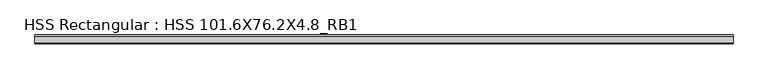
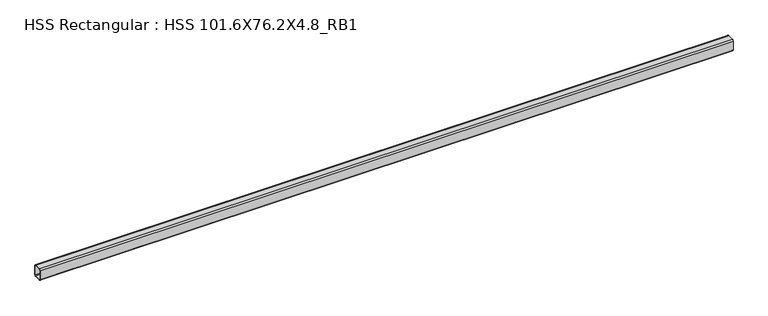
"""IFC4 building model written with IfcOpenShell, lengths in millimetres: beam geometry, HSS Rectangular : HSS 101.6X76.2X4.8_RB1."""

from ifc_helpers import new_model, si_unit, point, frame, frame_2d, origin, place, context, project, spatial, polyline, circle_curve, trimmed, segment, composite_curve, outline, extrude, source, transform, mapped, element, save


def hss_rectangular_hss_101_6x76_2x4_8_rb1_16b1f6f2(model_context):
    return source(origin(), model_context, "Body", "SweptSolid", [
        extrude(outline(composite_curve([segment(polyline([(38.1, 41.275), (38.1, -41.275)]), True, "CONTINUOUS"), segment(trimmed(circle_curve(frame_2d((28.575, -41.275)), 9.525), [point((38.1, -41.275))], [point((28.575, -50.8))], False, "CARTESIAN"), True, "CONTINUOUS"), segment(polyline([(28.575, -50.8), (-28.575, -50.8)]), True, "CONTINUOUS"), segment(trimmed(circle_curve(frame_2d((-28.575, -41.275)), 9.525), [point((-28.575, -50.8))], [point((-38.1, -41.275))], False, "CARTESIAN"), True, "CONTINUOUS"), segment(polyline([(-38.1, -41.275), (-38.1, 41.275)]), True, "CONTINUOUS"), segment(trimmed(circle_curve(frame_2d((-28.575, 41.275)), 9.525), [point((-38.1, 41.275))], [point((-28.575, 50.8))], False, "CARTESIAN"), True, "CONTINUOUS"), segment(polyline([(-28.575, 50.8), (28.575, 50.8)]), True, "CONTINUOUS"), segment(trimmed(circle_curve(frame_2d((28.575, 41.275)), 9.525), [point((28.575, 50.8))], [point((38.1, 41.275))], False, "CARTESIAN"), True, "CONTINUOUS")], self_intersect=False), holes=[composite_curve([segment(trimmed(circle_curve(frame_2d((-28.575, 41.275)), 4.7625), [point((-28.575, 46.0375))], [point((-33.3375, 41.275))], True, "CARTESIAN"), True, "CONTINUOUS"), segment(polyline([(-33.3375, 41.275), (-33.3375, -41.275)]), True, "CONTINUOUS"), segment(trimmed(circle_curve(frame_2d((-28.575, -41.275)), 4.7625), [point((-33.3375, -41.275))], [point((-28.575, -46.0375))], True, "CARTESIAN"), True, "CONTINUOUS"), segment(polyline([(-28.575, -46.0375), (28.575, -46.0375)]), True, "CONTINUOUS"), segment(trimmed(circle_curve(frame_2d((28.575, -41.275)), 4.7625), [point((28.575, -46.0375))], [point((33.3375, -41.275))], True, "CARTESIAN"), True, "CONTINUOUS"), segment(polyline([(33.3375, -41.275), (33.3375, 41.275)]), True, "CONTINUOUS"), segment(trimmed(circle_curve(frame_2d((28.575, 41.275)), 4.7625), [point((33.3375, 41.275))], [point((28.575, 46.0375))], True, "CARTESIAN"), True, "CONTINUOUS"), segment(polyline([(28.575, 46.0375), (-28.575, 46.0375)]), True, "CONTINUOUS")], self_intersect=False)]), frame((-7493.3247032, 0.0, 0.0), z_axis=(1.0, 0.0, 0.0), x_axis=(0.0, 1.0, 0.0)), (0.0, 0.0, 1.0), 5980.3759919),
    ])


if __name__ == "__main__":
    model = new_model("IFC4")
    model_context = context("Model", 3, world=origin())
    ifc_project = project(units=[si_unit("LENGTHUNIT", "METRE", prefix="MILLI")], contexts=[model_context])
    site = spatial("IfcSite", under=ifc_project)
    building = spatial("IfcBuilding", under=site)
    placement = place(None, origin())
    hss_rectangular_hss_101_6x76_2x4_8_rb1_shape = hss_rectangular_hss_101_6x76_2x4_8_rb1_16b1f6f2(model_context)
    element("IfcBeam", 1, ObjectType="HSS Rectangular : HSS 101.6X76.2X4.8_RB1", at=placement, inside=building, context=model_context, shape_type="MappedRepresentation", body=[
        mapped(hss_rectangular_hss_101_6x76_2x4_8_rb1_shape, transform((0.0, 0.0, 0.0), x_axis=(1.0, 0.0, 0.0), y_axis=(0.0, 1.0, 0.0), z_axis=(0.0, 0.0, 1.0))),
    ])
    save(model, "model.ifc")

# Revit data of these elements
# Type "HSS Rectangular : HSS 101.6X76.2X4.8_RB1"
#   Section Name Key = "HSS 4X3X3/16"
#   Assembly Code = "B10"
#   Width = 7.62 cm
#   Wall Nominal Thickness = 0.4763 cm
#   Wall Design Thickness = 0.442 cm
#   Torsional Moment of Inertia = 260.561 cm⁴
#   Torsional Modulus = 61.2876 cm³
#   Section Area = 14.4516 cm²
#   Plastic Modulus weak axis = 40.3122 cm³
#   Plastic Modulus strong axis = 49.1612 cm³
#   Perimeter = 0.881482 m²/m
#   Outer Fillet = 0.9525 cm
#   Nominal Weight = 12.1285 kgf/m
#   Moment of Inertia weak axis = 131.529 cm⁴
#   Moment of Inertia strong axis = 205.202 cm⁴
#   Inner Fillet = 0.4763 cm
#   Height = 10.16 cm
#   Elastic Modulus weak axis = 34.4128 cm³
#   Elastic Modulus strong axis = 40.476 cm³
#   Centroid Vertical = 5.08 cm
#   Centroid Horizontal = 3.81 cm
#   Length [instance default] = 1524 mm
#   Structural Material [instance default] = Steel ASTM A500, Grade B, Rectangular and Square
#   Principal Axes Angle = 0
# Element 1 (IfcBeam, "HSS Rectangular : HSS 101.6X76.2X4.8_RB1")
#   Structural Material = Steel ASTM A992
#   Materials on its faces: "Steel ASTM A992"
# Materials
#   "Steel ASTM A500, Grade B, Rectangular and Square": class "Metal", colour RGB 199 199 199, transparency 0, Description = "Carbon steel", Cost = 0
#   "Steel ASTM A992": class "Metal", colour RGB 199 199 199, transparency 0, Description = "Structural steel 50ksi", Cost = 0
